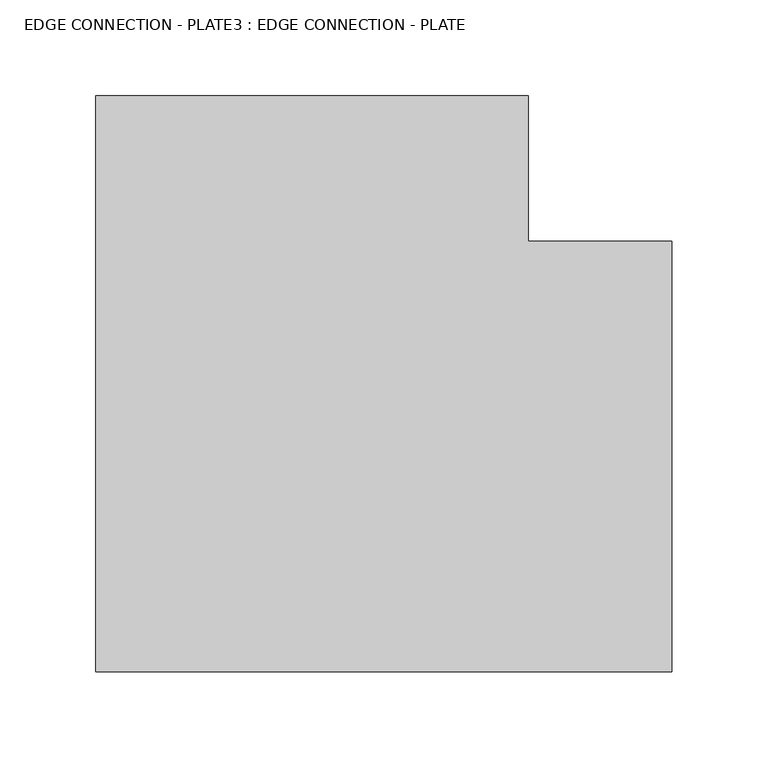
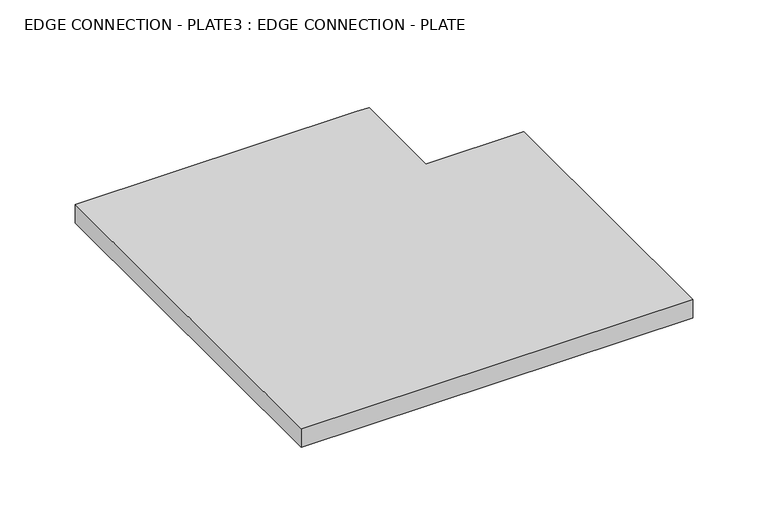
"""IFC4 building model written with IfcOpenShell, lengths in millimetres: fastener geometry, EDGE CONNECTION - PLATE3 : EDGE CONNECTION - PLATE."""

from ifc_helpers import new_model, si_unit, frame, origin, place, context, project, spatial, polyline, outline, extrude, source, transform, mapped, element, save


def edge_connection_plate3_edge_connection_plate_93e39276(model_context):
    return source(origin(), model_context, "Body", "SweptSolid", [
        extrude(outline(polyline([(-30642.9971664, -7594.7960995), (-30942.9971664, -7594.7960995), (-30942.9971664, -7294.7960995), (-30727.8591664, -7294.7960995), (-30717.8591664, -7294.7960995), (-30717.8591664, -7370.3260995), (-30642.9971664, -7370.3260995), (-30642.9971664, -7380.3260995), (-30642.9971664, -7594.7960995)])), frame((0.0, 0.0, 200.0), z_axis=(0.0, 0.0, 1.0), x_axis=(1.0, 0.0, 0.0)), (0.0, 0.0, 1.0), 15.0),
    ])


if __name__ == "__main__":
    model = new_model("IFC4")
    model_context = context("Model", 3, world=origin())
    ifc_project = project(units=[si_unit("LENGTHUNIT", "METRE", prefix="MILLI")], contexts=[model_context])
    site = spatial("IfcSite", under=ifc_project)
    building = spatial("IfcBuilding", under=site)
    placement = place(None, origin())
    edge_connection_plate3_edge_connection_plate_shape = edge_connection_plate3_edge_connection_plate_93e39276(model_context)
    element("IfcFastener", 1, ObjectType="EDGE CONNECTION - PLATE3 : EDGE CONNECTION - PLATE", at=placement, inside=building, context=model_context, shape_type="MappedRepresentation", body=[
        mapped(edge_connection_plate3_edge_connection_plate_shape, transform((0.0, 0.0, 0.0), x_axis=(1.0, 0.0, 0.0), y_axis=(0.0, 1.0, 0.0), z_axis=(0.0, 0.0, 1.0))),
    ])
    save(model, "model.ifc")
